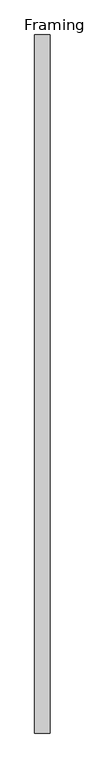
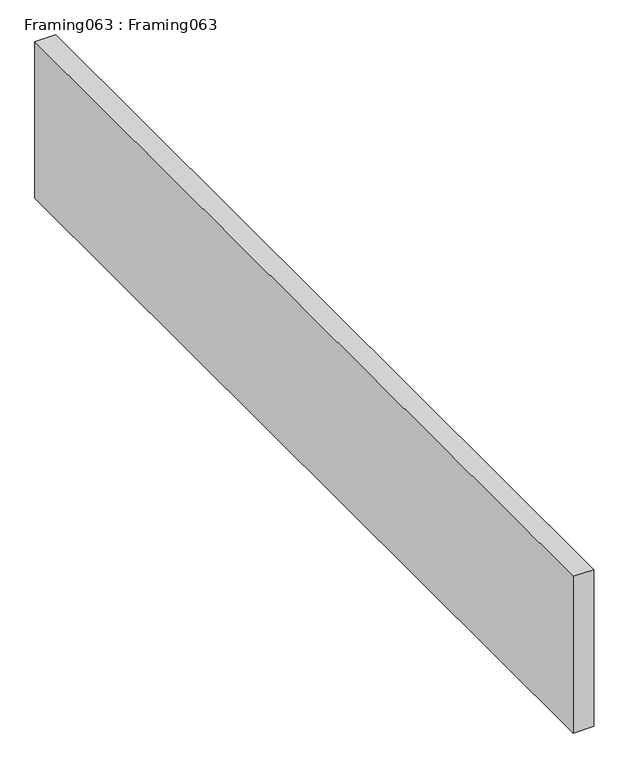
"""IFC4 building model written with IfcOpenShell, lengths in millimetres: proxy geometry, Framing063 : Framing063."""

from ifc_helpers import new_model, si_unit, frame, origin, place, context, project, spatial, polyline, outline, extrude, source, transform, mapped, element, save


def framing063_framing063_58675b7e(model_context):
    return source(origin(), model_context, "Body", "SweptSolid", [
        extrude(outline(polyline([(-574.1519086, -1052.8906574), (-618.6019086, -1052.8906574), (-618.6019086, 947.1093426), (-574.1519086, 947.1093426), (-574.1519086, -1052.8906574)])), frame((0.0, 0.0, 42134.105552), z_axis=(0.0, 0.0, 1.0), x_axis=(1.0, 0.0, 0.0)), (0.0, 0.0, 1.0), 355.2981173),
    ])


if __name__ == "__main__":
    model = new_model("IFC4")
    model_context = context("Model", 3, world=origin())
    ifc_project = project(units=[si_unit("LENGTHUNIT", "METRE", prefix="MILLI")], contexts=[model_context])
    site = spatial("IfcSite", under=ifc_project)
    building = spatial("IfcBuilding", under=site)
    placement = place(None, origin())
    framing063_framing063_shape = framing063_framing063_58675b7e(model_context)
    element("IfcBuildingElementProxy", 1, Name="Framing063 : Framing063", ObjectType="Framing063 : Framing063", at=placement, inside=building, context=model_context, shape_type="MappedRepresentation", body=[
        mapped(framing063_framing063_shape, transform((0.0, 0.0, 0.0), x_axis=(1.0, 0.0, 0.0), y_axis=(0.0, 1.0, 0.0), z_axis=(0.0, 0.0, 1.0))),
    ])
    save(model, "model.ifc")

# Revit data of these elements
# Type "Framing063 : Framing063"
#   NameOverride = "Framing063"
# Element 1 (IfcBuildingElementProxy, "Framing063 : Framing063")
#   Materials on its faces: "WOOD FRAMING (SEE STRUCT DWGS)"
# Materials
#   "WOOD FRAMING (SEE STRUCT DWGS)": class "Unassigned", colour RGB 224 188 168, transparency 0, Cost = 0
